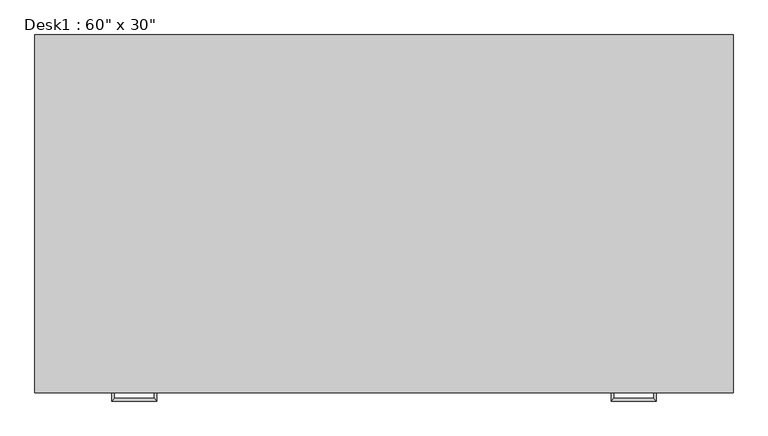
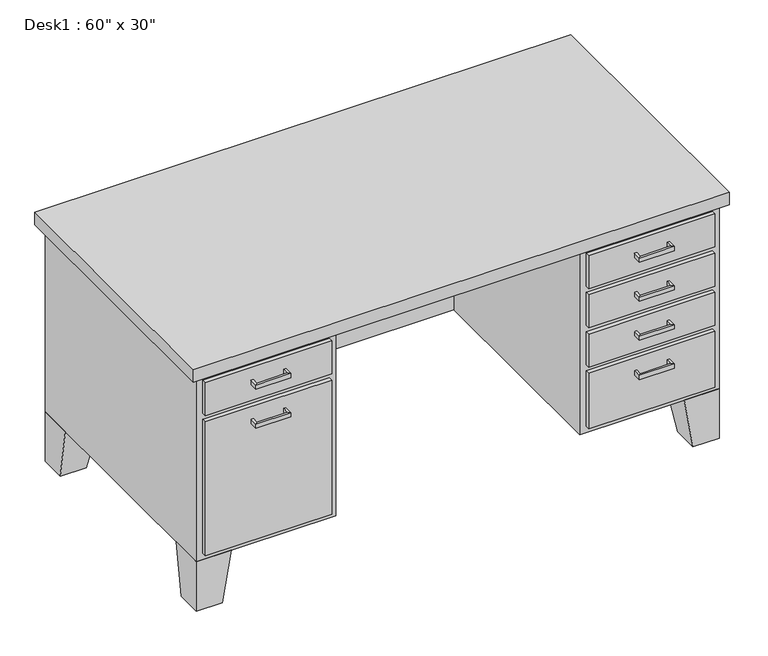
"""IFC4 building model written with IfcOpenShell, lengths in millimetres: furniture geometry."""

from ifc_helpers import new_model, si_unit, frame, origin, place, context, project, spatial, polyline, outline, extrude, faceted_brep, source, transform, mapped, element, save


def furniture_013ab306(model_context):
    return source(origin(), model_context, "Body", "SolidModel", [
        extrude(outline(polyline([(19.05, 0.0), (387.35, 0.0), (387.35, -12.7), (19.05, -12.7), (19.05, 0.0)])), frame((0.0, 0.0, 603.25), z_axis=(0.0, 0.0, 1.0), x_axis=(1.0, 0.0, 0.0)), (0.0, 0.0, 1.0), 101.6),
        extrude(outline(polyline([(19.05, 0.0), (387.35, 0.0), (387.35, -12.7), (19.05, -12.7), (19.05, 0.0)])), frame((0.0, 0.0, 171.45), z_axis=(0.0, 0.0, 1.0), x_axis=(1.0, 0.0, 0.0)), (0.0, 0.0, 1.0), 412.75),
        extrude(outline(polyline([(1136.65, 0.0), (1504.95, 0.0), (1504.95, -12.7), (1136.65, -12.7), (1136.65, 0.0)])), frame((0.0, 0.0, 603.25), z_axis=(0.0, 0.0, 1.0), x_axis=(1.0, 0.0, 0.0)), (0.0, 0.0, 1.0), 101.6),
        extrude(outline(polyline([(1136.65, 0.0), (1504.95, 0.0), (1504.95, -12.7), (1136.65, -12.7), (1136.65, 0.0)])), frame((0.0, 0.0, 171.45), z_axis=(0.0, 0.0, 1.0), x_axis=(1.0, 0.0, 0.0)), (0.0, 0.0, 1.0), 171.45),
        extrude(outline(polyline([(1136.65, 0.0), (1504.95, 0.0), (1504.95, -12.7), (1136.65, -12.7), (1136.65, 0.0)])), frame((0.0, 0.0, 482.6), z_axis=(0.0, 0.0, 1.0), x_axis=(1.0, 0.0, 0.0)), (0.0, 0.0, 1.0), 101.6),
        extrude(outline(polyline([(1136.65, 0.0), (1504.95, 0.0), (1504.95, -12.7), (1136.65, -12.7), (1136.65, 0.0)])), frame((0.0, 0.0, 361.95), z_axis=(0.0, 0.0, 1.0), x_axis=(1.0, 0.0, 0.0)), (0.0, 0.0, 1.0), 101.6),
        faceted_brep([(101.6, 0.0, 152.4), (101.6, 101.6, 152.4), (0.0, 101.6, 152.4), (0.0, 0.0, 152.4), (76.2, 0.0, 0.0), (0.0, 0.0, 0.0), (0.0, 76.2, 0.0), (76.2, 76.2, 0.0)], [[[0, 1, 2, 3]], [[4, 5, 6, 7]], [[4, 7, 1, 0]], [[7, 6, 2, 1]], [[6, 5, 3, 2]], [[5, 4, 0, 3]]]),
        faceted_brep([(101.6, 762.0, 152.4), (0.0, 762.0, 152.4), (0.0, 660.4, 152.4), (101.6, 660.4, 152.4), (76.2, 762.0, 0.0), (76.2, 685.8, 0.0), (0.0, 685.8, 0.0), (0.0, 762.0, 0.0)], [[[0, 1, 2, 3]], [[4, 5, 6, 7]], [[4, 7, 1, 0]], [[7, 6, 2, 1]], [[6, 5, 3, 2]], [[5, 4, 0, 3]]]),
        faceted_brep([(1422.4, 762.0, 152.4), (1422.4, 660.4, 152.4), (1524.0, 660.4, 152.4), (1524.0, 762.0, 152.4), (1447.8, 762.0, 0.0), (1524.0, 762.0, 0.0), (1524.0, 685.8, 0.0), (1447.8, 685.8, 0.0)], [[[0, 1, 2, 3]], [[4, 5, 6, 7]], [[4, 7, 1, 0]], [[7, 6, 2, 1]], [[6, 5, 3, 2]], [[5, 4, 0, 3]]]),
        faceted_brep([(1422.4, 0.0, 152.4), (1524.0, 0.0, 152.4), (1524.0, 101.6, 152.4), (1422.4, 101.6, 152.4), (1447.8, 0.0, 0.0), (1447.8, 76.2, 0.0), (1524.0, 76.2, 0.0), (1524.0, 0.0, 0.0)], [[[0, 1, 2, 3]], [[4, 5, 6, 7]], [[4, 7, 1, 0]], [[7, 6, 2, 1]], [[6, 5, 3, 2]], [[5, 4, 0, 3]]]),
        extrude(outline(polyline([(-19.05, -19.05), (-19.05, 781.05), (1543.05, 781.05), (1543.05, -19.05), (-19.05, -19.05)])), frame((0.0, 0.0, 723.9), z_axis=(0.0, 0.0, 1.0), x_axis=(1.0, 0.0, 0.0)), (0.0, 0.0, 1.0), 38.1),
        extrude(outline(polyline([(1117.6, 0.0), (1117.6, 635.0), (406.4, 635.0), (406.4, 0.0), (0.0, 0.0), (0.0, 762.0), (1524.0, 762.0), (1524.0, 0.0), (1117.6, 0.0)])), frame((0.0, 0.0, 152.4), z_axis=(0.0, 0.0, 1.0), x_axis=(1.0, 0.0, 0.0)), (0.0, 0.0, 1.0), 571.5),
        faceted_brep([(158.75, -12.7, 546.1), (158.75, -12.7, 533.4), (152.4, -12.7, 533.4), (152.4, -12.7, 546.1), (158.75, -31.75, 546.1), (158.75, -31.75, 533.4), (152.4, -38.1, 533.4), (152.4, -38.1, 546.1), (247.65, -31.75, 546.1), (247.65, -31.75, 533.4), (254.0, -38.1, 533.4), (254.0, -38.1, 546.1), (247.65, -12.7, 546.1), (254.0, -12.7, 546.1), (254.0, -12.7, 533.4), (247.65, -12.7, 533.4)], [[[0, 1, 2, 3]], [[1, 0, 4, 5]], [[2, 1, 5, 6]], [[3, 2, 6, 7]], [[0, 3, 7, 4]], [[5, 4, 8, 9]], [[6, 5, 9, 10]], [[7, 6, 10, 11]], [[4, 7, 11, 8]], [[12, 13, 14, 15]], [[9, 8, 12, 15]], [[10, 9, 15, 14]], [[11, 10, 14, 13]], [[8, 11, 13, 12]]]),
        faceted_brep([(158.75, -12.7, 666.75), (158.75, -12.7, 654.05), (152.4, -12.7, 654.05), (152.4, -12.7, 666.75), (158.75, -31.75, 666.75), (158.75, -31.75, 654.05), (152.4, -38.1, 654.05), (152.4, -38.1, 666.75), (247.65, -31.75, 666.75), (247.65, -31.75, 654.05), (254.0, -38.1, 654.05), (254.0, -38.1, 666.75), (247.65, -12.7, 666.75), (254.0, -12.7, 666.75), (254.0, -12.7, 654.05), (247.65, -12.7, 654.05)], [[[0, 1, 2, 3]], [[1, 0, 4, 5]], [[2, 1, 5, 6]], [[3, 2, 6, 7]], [[0, 3, 7, 4]], [[5, 4, 8, 9]], [[6, 5, 9, 10]], [[7, 6, 10, 11]], [[4, 7, 11, 8]], [[12, 13, 14, 15]], [[9, 8, 12, 15]], [[10, 9, 15, 14]], [[11, 10, 14, 13]], [[8, 11, 13, 12]]]),
        faceted_brep([(1365.25, -12.7, 304.8), (1371.6, -12.7, 304.8), (1371.6, -12.7, 292.1), (1365.25, -12.7, 292.1), (1365.25, -31.75, 304.8), (1371.6, -38.1, 304.8), (1371.6, -38.1, 292.1), (1365.25, -31.75, 292.1), (1276.35, -31.75, 304.8), (1270.0, -38.1, 304.8), (1270.0, -38.1, 292.1), (1276.35, -31.75, 292.1), (1276.35, -12.7, 304.8), (1276.35, -12.7, 292.1), (1270.0, -12.7, 292.1), (1270.0, -12.7, 304.8)], [[[0, 1, 2, 3]], [[1, 0, 4, 5]], [[2, 1, 5, 6]], [[3, 2, 6, 7]], [[0, 3, 7, 4]], [[5, 4, 8, 9]], [[6, 5, 9, 10]], [[7, 6, 10, 11]], [[4, 7, 11, 8]], [[12, 13, 14, 15]], [[9, 8, 12, 15]], [[10, 9, 15, 14]], [[11, 10, 14, 13]], [[8, 11, 13, 12]]]),
        faceted_brep([(1365.25, -12.7, 425.45), (1371.6, -12.7, 425.45), (1371.6, -12.7, 412.75), (1365.25, -12.7, 412.75), (1365.25, -31.75, 425.45), (1371.6, -38.1, 425.45), (1371.6, -38.1, 412.75), (1365.25, -31.75, 412.75), (1276.35, -31.75, 425.45), (1270.0, -38.1, 425.45), (1270.0, -38.1, 412.75), (1276.35, -31.75, 412.75), (1276.35, -12.7, 425.45), (1276.35, -12.7, 412.75), (1270.0, -12.7, 412.75), (1270.0, -12.7, 425.45)], [[[0, 1, 2, 3]], [[1, 0, 4, 5]], [[2, 1, 5, 6]], [[3, 2, 6, 7]], [[0, 3, 7, 4]], [[5, 4, 8, 9]], [[6, 5, 9, 10]], [[7, 6, 10, 11]], [[4, 7, 11, 8]], [[12, 13, 14, 15]], [[9, 8, 12, 15]], [[10, 9, 15, 14]], [[11, 10, 14, 13]], [[8, 11, 13, 12]]]),
        faceted_brep([(1365.25, -12.7, 546.1), (1371.6, -12.7, 546.1), (1371.6, -12.7, 533.4), (1365.25, -12.7, 533.4), (1365.25, -31.75, 546.1), (1371.6, -38.1, 546.1), (1371.6, -38.1, 533.4), (1365.25, -31.75, 533.4), (1276.35, -31.75, 546.1), (1270.0, -38.1, 546.1), (1270.0, -38.1, 533.4), (1276.35, -31.75, 533.4), (1276.35, -12.7, 546.1), (1276.35, -12.7, 533.4), (1270.0, -12.7, 533.4), (1270.0, -12.7, 546.1)], [[[0, 1, 2, 3]], [[1, 0, 4, 5]], [[2, 1, 5, 6]], [[3, 2, 6, 7]], [[0, 3, 7, 4]], [[5, 4, 8, 9]], [[6, 5, 9, 10]], [[7, 6, 10, 11]], [[4, 7, 11, 8]], [[12, 13, 14, 15]], [[9, 8, 12, 15]], [[10, 9, 15, 14]], [[11, 10, 14, 13]], [[8, 11, 13, 12]]]),
        faceted_brep([(1365.25, -12.7, 666.75), (1371.6, -12.7, 666.75), (1371.6, -12.7, 654.05), (1365.25, -12.7, 654.05), (1365.25, -31.75, 666.75), (1371.6, -38.1, 666.75), (1371.6, -38.1, 654.05), (1365.25, -31.75, 654.05), (1276.35, -31.75, 666.75), (1270.0, -38.1, 666.75), (1270.0, -38.1, 654.05), (1276.35, -31.75, 654.05), (1276.35, -12.7, 666.75), (1276.35, -12.7, 654.05), (1270.0, -12.7, 654.05), (1270.0, -12.7, 666.75)], [[[0, 1, 2, 3]], [[1, 0, 4, 5]], [[2, 1, 5, 6]], [[3, 2, 6, 7]], [[0, 3, 7, 4]], [[5, 4, 8, 9]], [[6, 5, 9, 10]], [[7, 6, 10, 11]], [[4, 7, 11, 8]], [[12, 13, 14, 15]], [[9, 8, 12, 15]], [[10, 9, 15, 14]], [[11, 10, 14, 13]], [[8, 11, 13, 12]]]),
    ])


if __name__ == "__main__":
    model = new_model("IFC4")
    model_context = context("Model", 3, world=origin())
    ifc_project = project(units=[si_unit("LENGTHUNIT", "METRE", prefix="MILLI")], contexts=[model_context])
    site = spatial("IfcSite", under=ifc_project)
    building = spatial("IfcBuilding", under=site)
    placement = place(None, origin())
    furniture_shape = furniture_013ab306(model_context)
    element("IfcFurniture", 1, ObjectType="Desk1 : 60\" x 30\"", at=placement, inside=building, context=model_context, shape_type="MappedRepresentation", body=[
        mapped(furniture_shape, transform((0.0, 0.0, 0.0), x_axis=(1.0, 0.0, 0.0), y_axis=(0.0, 1.0, 0.0), z_axis=(0.0, 0.0, 1.0))),
    ])
    save(model, "model.ifc")

# Revit data of these elements
# Type "Desk1 : 60\" x 30\""
#   Assembly Code = "E2020200"
#   Depth = 2' - 6"
#   Height = 2' - 6"
#   Leg Height = 0' - 6"
#   Width = 5' - 0"
#   Body Material = Laminate, Ivory, Matte
#   Handle/Leg Material = Steel, Chrome Plated
#   Top Material = Cherry
#   Default Elevation = 0
# Element 1 (IfcFurniture, "Desk1 : 60\" x 30\"")
#   Materials on its faces: "Steel, Chrome Plated", "Laminate, Ivory, Matte", "Cherry"
# Materials
#   "Laminate, Ivory, Matte": class "Plastic", colour RGB 247 247 239, transparency 0, Description = "Plastic Laminate - Ivory, Matte", Cost = 0
#   "Steel, Chrome Plated": class "Metal", colour RGB 17 17 17, transparency 0, Description = "Chromiuim plated steel", Cost = 0
#   "Cherry": class "Wood", colour RGB 226 177 128, transparency 0, Description = "Prunus Serotina", Cost = 0
